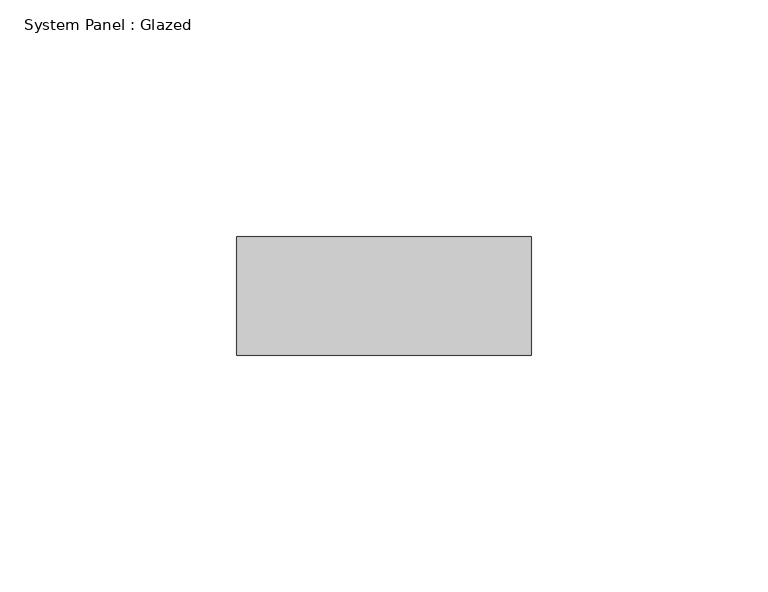
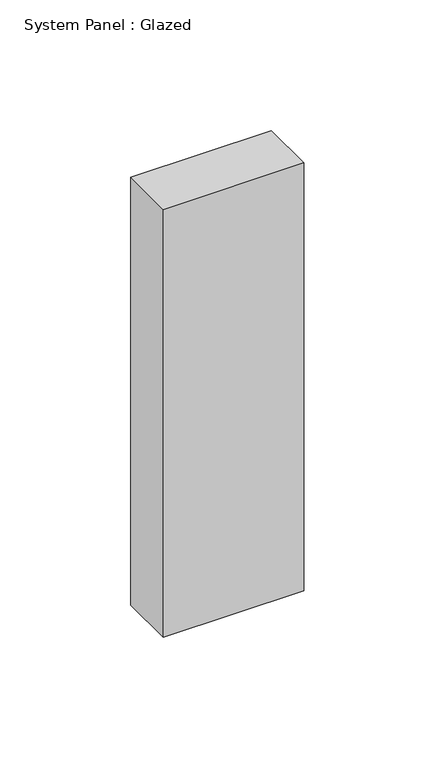
"""IFC4 building model written with IfcOpenShell, lengths in millimetres: plate geometry, System Panel : Glazed."""

from ifc_helpers import new_model, si_unit, origin, origin_with_axes, place, context, project, spatial, polyline, outline, extrude, source, transform, mapped, element, save


def system_panel_glazed_6880485c(model_context):
    return source(origin(), model_context, "Body", "SweptSolid", [
        extrude(outline(polyline([(31.120151, 24.5), (-31.120151, 24.5), (-31.120151, 49.5), (31.120151, 49.5), (31.120151, 24.5)])), origin_with_axes(), (0.0, 0.0, 1.0), 200.0),
    ])


if __name__ == "__main__":
    model = new_model("IFC4")
    model_context = context("Model", 3, world=origin())
    ifc_project = project(units=[si_unit("LENGTHUNIT", "METRE", prefix="MILLI")], contexts=[model_context])
    site = spatial("IfcSite", under=ifc_project)
    building = spatial("IfcBuilding", under=site)
    placement = place(None, origin())
    system_panel_glazed_shape = system_panel_glazed_6880485c(model_context)
    element("IfcPlate", 1, ObjectType="System Panel : Glazed", at=placement, inside=building, context=model_context, shape_type="MappedRepresentation", body=[
        mapped(system_panel_glazed_shape, transform((0.0, 0.0, 0.0), x_axis=(1.0, 0.0, 0.0), y_axis=(0.0, 1.0, 0.0), z_axis=(0.0, 0.0, 1.0))),
    ])
    save(model, "model.ifc")

# Revit data of these elements
# Element 1 (IfcPlate, "System Panel : Glazed")
#   Materials on its faces: "Glass"
# Materials
#   "Glass": class "Glass", colour RGB 218 227 224, transparency 0.85, Description = "Soda Lime Glass", Cost = 0
